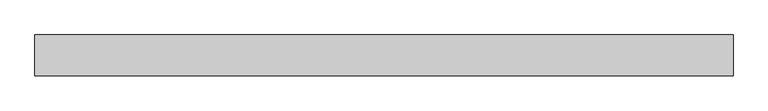
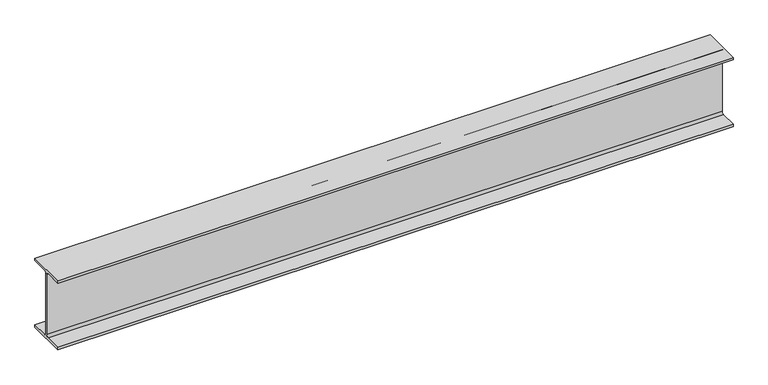
"""IFC4 building model written with IfcOpenShell, lengths in millimetres: beam geometry, Old_Steel Beam_H-KSD3502 : H_SB_ASB_H-250×125x6x9."""

from ifc_helpers import new_model, si_unit, point, frame, frame_2d, origin, place, context, project, spatial, polyline, circle_curve, trimmed, segment, composite_curve, outline, extrude, source, transform, mapped, element, save


def beam_9a7c615d(model_context):
    return source(origin(), model_context, "Body", "SweptSolid", [
        extrude(outline(composite_curve([segment(polyline([(82.5, -141.5), (82.5, -151.7), (-82.5, -151.7), (-82.5, -141.5), (-11.9, -141.5)]), True, "CONTINUOUS"), segment(trimmed(circle_curve(frame_2d((-11.9, -132.6)), 8.9), [point((-11.9, -141.5))], [point((-3.0, -132.6))], True, "CARTESIAN"), True, "CONTINUOUS"), segment(polyline([(-3.0, -132.6), (-3.0, 132.6)]), True, "CONTINUOUS"), segment(trimmed(circle_curve(frame_2d((-11.9, 132.6)), 8.9), [point((-3.0, 132.6))], [point((-11.9, 141.5))], True, "CARTESIAN"), True, "CONTINUOUS"), segment(polyline([(-11.9, 141.5), (-82.5, 141.5), (-82.5, 151.7), (82.5, 151.7), (82.5, 141.5), (11.9, 141.5)]), True, "CONTINUOUS"), segment(trimmed(circle_curve(frame_2d((11.9, 132.6)), 8.9), [point((11.9, 141.5))], [point((3.0, 132.6))], True, "CARTESIAN"), True, "CONTINUOUS"), segment(polyline([(3.0, 132.6), (3.0, -132.6)]), True, "CONTINUOUS"), segment(trimmed(circle_curve(frame_2d((11.9, -132.6)), 8.9), [point((3.0, -132.6))], [point((11.9, -141.5))], True, "CARTESIAN"), True, "CONTINUOUS"), segment(polyline([(11.9, -141.5), (82.5, -141.5)]), True, "CONTINUOUS")], self_intersect=False)), frame((-1404.7192363, 0.0, 0.0), z_axis=(1.0, 0.0, 0.0), x_axis=(0.0, 1.0, 0.0)), (0.0, 0.0, 1.0), 2809.5192866),
    ])


if __name__ == "__main__":
    model = new_model("IFC4")
    model_context = context("Model", 3, world=origin())
    ifc_project = project(units=[si_unit("LENGTHUNIT", "METRE", prefix="MILLI")], contexts=[model_context])
    site = spatial("IfcSite", under=ifc_project)
    building = spatial("IfcBuilding", under=site)
    placement = place(None, origin())
    beam_shape = beam_9a7c615d(model_context)
    element("IfcBeam", 1, ObjectType="Old_Steel Beam_H-KSD3502 : H_SB_ASB_H-250×125x6x9", at=placement, inside=building, context=model_context, shape_type="MappedRepresentation", body=[
        mapped(beam_shape, transform((0.0, 0.0, 0.0), x_axis=(1.0, 0.0, 0.0), y_axis=(0.0, 1.0, 0.0), z_axis=(0.0, 0.0, 1.0))),
    ])
    save(model, "model.ifc")

# Revit data of these elements
# Type "Old_Steel Beam_H-KSD3502 : H_SB_ASB_H-250×125x6x9"
#   Width = 12.5 cm
#   Web Thickness = 0.6 cm
#   Web Fillet = 1.2 cm
#   Warping Constant = 42539.8 cm⁶
#   Torsional Moment of Inertia = 7.8102 cm⁴
#   Torsional Modulus = 1.0 cm³
#   Section Area = 37.66 cm²
#   Plastic Modulus weak axis = 73.1 cm³
#   Plastic Modulus strong axis = 366.0 cm³
#   Perimeter = 0.97 m²/m
#   Nominal Weight = 29.60 kgf/m
#   Moment of Inertia weak axis = 294.00 cm⁴
#   Moment of Inertia strong axis = 4050.00 cm⁴
#   Height = 25.0 cm
#   Flange Thickness = 0.9 cm
#   Elastic Modulus weak axis = 47.0 cm³
#   Elastic Modulus strong axis = 324.0 cm³
#   Centroid Vertical = 12.5 cm
#   Centroid Horizontal = 6.25 cm
#   Length [instance default] = 1.5240 m
#   Structural Material [instance default] = Steel, 45-345
#   Assembly Code = ""
# Element 1 (IfcBeam, "Old_Steel Beam_H-KSD3502 : H_SB_ASB_H-250×125x6x9")
#   Structural Material = none
# Materials
#   "Steel, 45-345": class "Metal", colour RGB 189 187 185, transparency 0, Description = "Steel 345 MPa", Cost = 0
